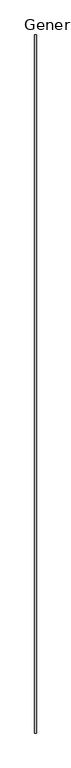
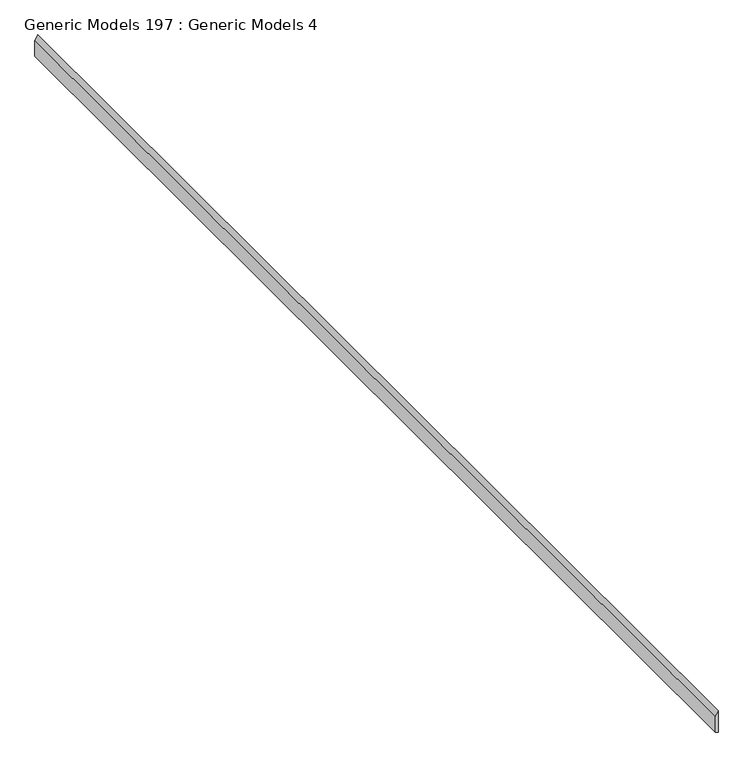
"""IFC4 building model written with IfcOpenShell, lengths in millimetres: proxy geometry, Generic Models 197 : Generic Models 4."""

from ifc_helpers import new_model, si_unit, frame, origin, place, context, project, spatial, polyline, outline, extrude, source, transform, mapped, element, save


def generic_models_197_generic_models_4_3d276085(model_context):
    return source(origin(), model_context, "Body", "SweptSolid", [
        extrude(outline(polyline([(126810.6253954, -8158.6536295), (126804.9103954, -8140.8736295), (126949.0984618, -8140.8736295), (126914.4742513, -8158.6536295), (126810.6253954, -8158.6536295)])), frame((0.0, -464.1230338, 0.0), z_axis=(0.0, 1.0, 0.0), x_axis=(0.0, 0.0, 1.0)), (0.0, 0.0, 1.0), 7518.4),
    ])


if __name__ == "__main__":
    model = new_model("IFC4")
    model_context = context("Model", 3, world=origin())
    ifc_project = project(units=[si_unit("LENGTHUNIT", "METRE", prefix="MILLI")], contexts=[model_context])
    site = spatial("IfcSite", under=ifc_project)
    building = spatial("IfcBuilding", under=site)
    placement = place(None, origin())
    generic_models_197_generic_models_4_shape = generic_models_197_generic_models_4_3d276085(model_context)
    element("IfcBuildingElementProxy", 1, Name="Generic Models 197 : Generic Models 4", ObjectType="Generic Models 197 : Generic Models 4", at=placement, inside=building, context=model_context, shape_type="MappedRepresentation", body=[
        mapped(generic_models_197_generic_models_4_shape, transform((0.0, 0.0, 0.0), x_axis=(1.0, 0.0, 0.0), y_axis=(0.0, 1.0, 0.0), z_axis=(0.0, 0.0, 1.0))),
    ])
    save(model, "model.ifc")

# Revit data of these elements
# Element 1 (IfcBuildingElementProxy, "Generic Models 197 : Generic Models 4")
#   Materials on its faces: "_7/8\" SMOOTH TROWEL EXTERIOR STUCCO (COLOR PER OWNER)"
# Materials
#   "_7/8\" SMOOTH TROWEL EXTERIOR STUCCO (COLOR PER OWNER)": class "Generic", colour RGB 233 233 233, transparency 0, Cost = 0
